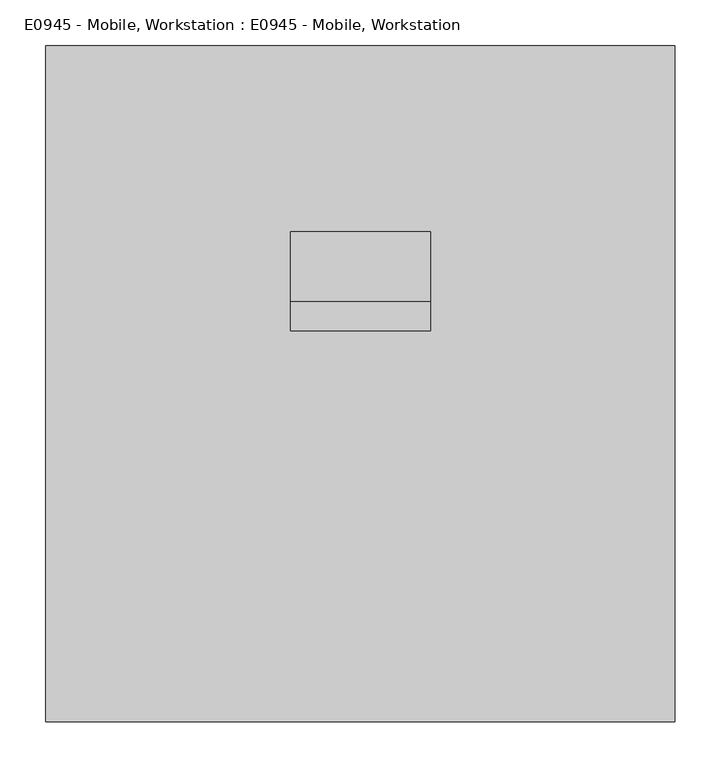
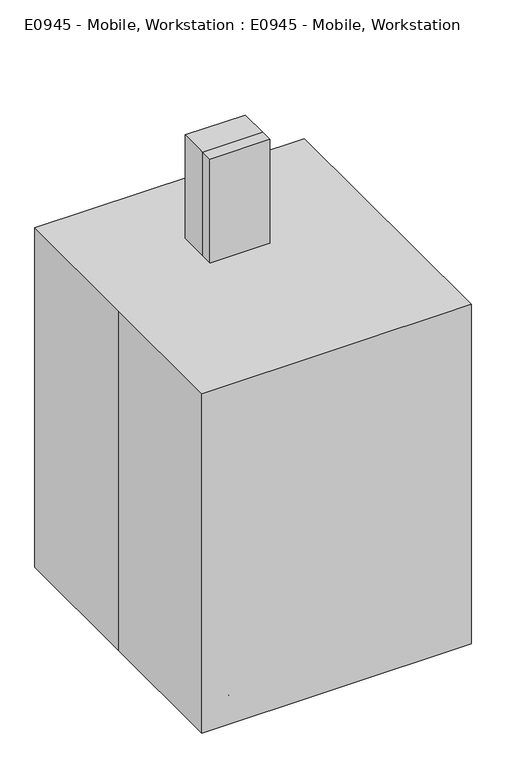
"""IFC4 building model written with IfcOpenShell, lengths in millimetres: proxy geometry, E0945 - Mobile, Workstation : E0945 - Mobile, Workstation."""

from ifc_helpers import new_model, si_unit, point, frame, frame_2d, origin, origin_with_axes, place, context, project, spatial, polyline, circle_curve, trimmed, segment, composite_curve, outline, extrude, faceted_brep, source, transform, mapped, element, save


def e0945_mobile_workstation_e0945_mobile_workstation_0c41a28f(model_context):
    return source(origin(), model_context, "Body", "SolidModel", [
        extrude(outline(polyline([(-196.85, 635.0), (58.0280886, 635.0), (58.0280886, 444.5), (-196.85, 609.6), (-196.85, 635.0)])), frame((57.15, 0.0, 0.0), z_axis=(1.0, 0.0, 0.0), x_axis=(0.0, 1.0, 0.0)), (0.0, 0.0, 1.0), 19.05),
        faceted_brep([(211.1375, -4.7625, 644.525), (211.1375, -4.7625, 639.7625), (211.1375, -255.5875, 639.7625), (211.1375, -255.5875, 644.525), (215.9, 0.0, 644.525), (215.9, -260.35, 644.525), (215.9, -260.35, 635.0), (215.9, 0.0, 635.0), (-211.1375, -255.5875, 639.7625), (-211.1375, -255.5875, 644.525), (-215.9, -260.35, 644.525), (-215.9, -260.35, 635.0), (-211.1375, -4.7625, 639.7625), (-211.1375, -4.7625, 644.525), (-215.9, 0.0, 644.525), (-215.9, 0.0, 635.0)], [[[0, 1, 2, 3]], [[4, 5, 6, 7]], [[3, 2, 8, 9]], [[6, 5, 10, 11]], [[9, 8, 12, 13]], [[11, 10, 14, 15]], [[1, 0, 13, 12]], [[5, 4, 14, 10], [0, 3, 9, 13]], [[4, 7, 15, 14]], [[7, 6, 11, 15]], [[2, 1, 12, 8]]]),
        extrude(outline(polyline([(-196.85, 635.0), (58.0280886, 635.0), (58.0280886, 444.5), (-196.85, 609.6), (-196.85, 635.0)])), frame((-76.2, 0.0, 0.0), z_axis=(1.0, 0.0, 0.0), x_axis=(0.0, 1.0, 0.0)), (0.0, 0.0, 1.0), 19.05),
        extrude(outline(polyline([(76.2, 89.7780886), (76.2, 58.0280886), (-76.2, 58.0280886), (-76.2, 89.7780886), (76.2, 89.7780886)])), frame((0.0, 0.0, 444.5), z_axis=(0.0, 0.0, 1.0), x_axis=(1.0, 0.0, 0.0)), (0.0, 0.0, 1.0), 749.3),
        extrude(outline(composite_curve([segment(polyline([(165.9780886, 1193.8), (165.9780886, 139.7), (62.2305834, 139.7)]), True, "CONTINUOUS"), segment(trimmed(circle_curve(frame_2d((29.5735373, 190.9359281)), 60.7585631), [point((62.2305834, 139.7))], [point((89.7780886, 182.7496596))], True, "CARTESIAN"), True, "CONTINUOUS"), segment(polyline([(89.7780886, 182.7496596), (89.7780886, 1193.8), (165.9780886, 1193.8)]), True, "CONTINUOUS")], self_intersect=False)), frame((-76.2, 0.0, 0.0), z_axis=(1.0, 0.0, 0.0), x_axis=(0.0, 1.0, 0.0)), (0.0, 0.0, 1.0), 152.4),
        extrude(outline(composite_curve([segment(trimmed(circle_curve(frame_2d((-215.9, 257.2471418)), 9.525), [point((-206.375, 257.2471418))], [point((-225.425, 257.2471418))], False, "CARTESIAN"), True, "CONTINUOUS"), segment(trimmed(circle_curve(frame_2d((-215.9, 257.2471418)), 9.525), [point((-225.425, 257.2471418))], [point((-206.375, 257.2471418))], False, "CARTESIAN"), True, "CONTINUOUS")], self_intersect=False)), frame((0.0, 0.0, 38.9774203), z_axis=(0.0, 0.0, 1.0), x_axis=(1.0, 0.0, 0.0)), (0.0, 0.0, 1.0), 49.9225797),
        extrude(outline(composite_curve([segment(trimmed(circle_curve(frame_2d((260.2876401, 38.1)), 38.1), [point((298.3876401, 38.1))], [point((222.1876401, 38.1))], False, "CARTESIAN"), True, "CONTINUOUS"), segment(trimmed(circle_curve(frame_2d((260.2876401, 38.1)), 38.1), [point((222.1876401, 38.1))], [point((298.3876401, 38.1))], False, "CARTESIAN"), True, "CONTINUOUS")], self_intersect=False)), frame((-206.375, 0.0, 0.0), z_axis=(1.0, 0.0, 0.0), x_axis=(0.0, 1.0, 0.0)), (0.0, 0.0, 1.0), 9.525),
        extrude(outline(composite_curve([segment(trimmed(circle_curve(frame_2d((260.35, 38.1)), 19.05), [point((279.4, 38.1))], [point((241.3, 38.1))], False, "CARTESIAN"), True, "CONTINUOUS"), segment(trimmed(circle_curve(frame_2d((260.35, 38.1)), 19.05), [point((241.3, 38.1))], [point((279.4, 38.1))], False, "CARTESIAN"), True, "CONTINUOUS")], self_intersect=False)), frame((-225.425, 0.0, 0.0), z_axis=(1.0, 0.0, 0.0), x_axis=(0.0, 1.0, 0.0)), (0.0, 0.0, 1.0), 19.05),
        extrude(outline(composite_curve([segment(trimmed(circle_curve(frame_2d((260.2876401, 38.1)), 38.1), [point((298.3876401, 38.1))], [point((222.1876401, 38.1))], False, "CARTESIAN"), True, "CONTINUOUS"), segment(trimmed(circle_curve(frame_2d((260.2876401, 38.1)), 38.1), [point((222.1876401, 38.1))], [point((298.3876401, 38.1))], False, "CARTESIAN"), True, "CONTINUOUS")], self_intersect=False)), frame((-234.95, 0.0, 0.0), z_axis=(1.0, 0.0, 0.0), x_axis=(0.0, 1.0, 0.0)), (0.0, 0.0, 1.0), 9.525),
        extrude(outline(composite_curve([segment(trimmed(circle_curve(frame_2d((-215.9, -257.2471418)), 9.525), [point((-206.375, -257.2471418))], [point((-225.425, -257.2471418))], False, "CARTESIAN"), True, "CONTINUOUS"), segment(trimmed(circle_curve(frame_2d((-215.9, -257.2471418)), 9.525), [point((-225.425, -257.2471418))], [point((-206.375, -257.2471418))], False, "CARTESIAN"), True, "CONTINUOUS")], self_intersect=False)), frame((0.0, 0.0, 38.9774203), z_axis=(0.0, 0.0, 1.0), x_axis=(1.0, 0.0, 0.0)), (0.0, 0.0, 1.0), 49.9225797),
        extrude(outline(composite_curve([segment(trimmed(circle_curve(frame_2d((-260.2876401, 38.1)), 38.1), [point((-298.3876401, 38.1))], [point((-222.1876401, 38.1))], False, "CARTESIAN"), True, "CONTINUOUS"), segment(trimmed(circle_curve(frame_2d((-260.2876401, 38.1)), 38.1), [point((-222.1876401, 38.1))], [point((-298.3876401, 38.1))], False, "CARTESIAN"), True, "CONTINUOUS")], self_intersect=False)), frame((-206.375, 0.0, 0.0), z_axis=(1.0, 0.0, 0.0), x_axis=(0.0, 1.0, 0.0)), (0.0, 0.0, 1.0), 9.525),
        extrude(outline(composite_curve([segment(trimmed(circle_curve(frame_2d((-260.35, 38.1)), 19.05), [point((-279.4, 38.1))], [point((-241.3, 38.1))], False, "CARTESIAN"), True, "CONTINUOUS"), segment(trimmed(circle_curve(frame_2d((-260.35, 38.1)), 19.05), [point((-241.3, 38.1))], [point((-279.4, 38.1))], False, "CARTESIAN"), True, "CONTINUOUS")], self_intersect=False)), frame((-225.425, 0.0, 0.0), z_axis=(1.0, 0.0, 0.0), x_axis=(0.0, 1.0, 0.0)), (0.0, 0.0, 1.0), 19.05),
        extrude(outline(composite_curve([segment(trimmed(circle_curve(frame_2d((-260.2876401, 38.1)), 38.1), [point((-298.3876401, 38.1))], [point((-222.1876401, 38.1))], False, "CARTESIAN"), True, "CONTINUOUS"), segment(trimmed(circle_curve(frame_2d((-260.2876401, 38.1)), 38.1), [point((-222.1876401, 38.1))], [point((-298.3876401, 38.1))], False, "CARTESIAN"), True, "CONTINUOUS")], self_intersect=False)), frame((-234.95, 0.0, 0.0), z_axis=(1.0, 0.0, 0.0), x_axis=(0.0, 1.0, 0.0)), (0.0, 0.0, 1.0), 9.525),
        extrude(outline(composite_curve([segment(trimmed(circle_curve(frame_2d((215.9, 257.2471418)), 9.525), [point((206.375, 257.2471418))], [point((225.425, 257.2471418))], False, "CARTESIAN"), True, "CONTINUOUS"), segment(trimmed(circle_curve(frame_2d((215.9, 257.2471418)), 9.525), [point((225.425, 257.2471418))], [point((206.375, 257.2471418))], False, "CARTESIAN"), True, "CONTINUOUS")], self_intersect=False)), frame((0.0, 0.0, 38.9774203), z_axis=(0.0, 0.0, 1.0), x_axis=(1.0, 0.0, 0.0)), (0.0, 0.0, 1.0), 49.9225797),
        extrude(outline(composite_curve([segment(trimmed(circle_curve(frame_2d((260.2876401, 38.1)), 38.1), [point((298.3876401, 38.1))], [point((222.1876401, 38.1))], False, "CARTESIAN"), True, "CONTINUOUS"), segment(trimmed(circle_curve(frame_2d((260.2876401, 38.1)), 38.1), [point((222.1876401, 38.1))], [point((298.3876401, 38.1))], False, "CARTESIAN"), True, "CONTINUOUS")], self_intersect=False)), frame((196.85, 0.0, 0.0), z_axis=(1.0, 0.0, 0.0), x_axis=(0.0, 1.0, 0.0)), (0.0, 0.0, 1.0), 9.525),
        extrude(outline(composite_curve([segment(trimmed(circle_curve(frame_2d((260.35, 38.1)), 19.05), [point((279.4, 38.1))], [point((241.3, 38.1))], False, "CARTESIAN"), True, "CONTINUOUS"), segment(trimmed(circle_curve(frame_2d((260.35, 38.1)), 19.05), [point((241.3, 38.1))], [point((279.4, 38.1))], False, "CARTESIAN"), True, "CONTINUOUS")], self_intersect=False)), frame((206.375, 0.0, 0.0), z_axis=(1.0, 0.0, 0.0), x_axis=(0.0, 1.0, 0.0)), (0.0, 0.0, 1.0), 19.05),
        extrude(outline(composite_curve([segment(trimmed(circle_curve(frame_2d((260.2876401, 38.1)), 38.1), [point((298.3876401, 38.1))], [point((222.1876401, 38.1))], False, "CARTESIAN"), True, "CONTINUOUS"), segment(trimmed(circle_curve(frame_2d((260.2876401, 38.1)), 38.1), [point((222.1876401, 38.1))], [point((298.3876401, 38.1))], False, "CARTESIAN"), True, "CONTINUOUS")], self_intersect=False)), frame((225.425, 0.0, 0.0), z_axis=(1.0, 0.0, 0.0), x_axis=(0.0, 1.0, 0.0)), (0.0, 0.0, 1.0), 9.525),
        extrude(outline(composite_curve([segment(trimmed(circle_curve(frame_2d((215.9, -257.2471418)), 9.525), [point((206.375, -257.2471418))], [point((225.425, -257.2471418))], False, "CARTESIAN"), True, "CONTINUOUS"), segment(trimmed(circle_curve(frame_2d((215.9, -257.2471418)), 9.525), [point((225.425, -257.2471418))], [point((206.375, -257.2471418))], False, "CARTESIAN"), True, "CONTINUOUS")], self_intersect=False)), frame((0.0, 0.0, 38.9774203), z_axis=(0.0, 0.0, 1.0), x_axis=(1.0, 0.0, 0.0)), (0.0, 0.0, 1.0), 49.9225797),
        extrude(outline(composite_curve([segment(trimmed(circle_curve(frame_2d((-260.2876401, 38.1)), 38.1), [point((-298.3876401, 38.1))], [point((-222.1876401, 38.1))], False, "CARTESIAN"), True, "CONTINUOUS"), segment(trimmed(circle_curve(frame_2d((-260.2876401, 38.1)), 38.1), [point((-222.1876401, 38.1))], [point((-298.3876401, 38.1))], False, "CARTESIAN"), True, "CONTINUOUS")], self_intersect=False)), frame((196.85, 0.0, 0.0), z_axis=(1.0, 0.0, 0.0), x_axis=(0.0, 1.0, 0.0)), (0.0, 0.0, 1.0), 9.525),
        extrude(outline(composite_curve([segment(trimmed(circle_curve(frame_2d((-260.35, 38.1)), 19.05), [point((-279.4, 38.1))], [point((-241.3, 38.1))], False, "CARTESIAN"), True, "CONTINUOUS"), segment(trimmed(circle_curve(frame_2d((-260.35, 38.1)), 19.05), [point((-241.3, 38.1))], [point((-279.4, 38.1))], False, "CARTESIAN"), True, "CONTINUOUS")], self_intersect=False)), frame((206.375, 0.0, 0.0), z_axis=(1.0, 0.0, 0.0), x_axis=(0.0, 1.0, 0.0)), (0.0, 0.0, 1.0), 19.05),
        extrude(outline(composite_curve([segment(trimmed(circle_curve(frame_2d((-260.2876401, 38.1)), 38.1), [point((-298.3876401, 38.1))], [point((-222.1876401, 38.1))], False, "CARTESIAN"), True, "CONTINUOUS"), segment(trimmed(circle_curve(frame_2d((-260.2876401, 38.1)), 38.1), [point((-222.1876401, 38.1))], [point((-298.3876401, 38.1))], False, "CARTESIAN"), True, "CONTINUOUS")], self_intersect=False)), frame((225.425, 0.0, 0.0), z_axis=(1.0, 0.0, 0.0), x_axis=(0.0, 1.0, 0.0)), (0.0, 0.0, 1.0), 9.525),
        extrude(outline(composite_curve([segment(polyline([(93.9865963, 192.9187071), (176.6628647, 292.6165602)]), True, "CONTINUOUS"), segment(trimmed(circle_curve(frame_2d((215.7665691, 260.189098)), 50.8), [point((176.6628647, 292.6165602))], [point((254.8702735, 227.7616359))], False, "CARTESIAN"), True, "CONTINUOUS"), segment(polyline([(254.8702735, 227.7616359), (152.4, 104.1945414), (152.4, -104.1945414), (254.8702735, -227.7616359)]), True, "CONTINUOUS"), segment(trimmed(circle_curve(frame_2d((215.7665691, -260.189098)), 50.8), [point((254.8702735, -227.7616359))], [point((176.6628647, -292.6165602))], False, "CARTESIAN"), True, "CONTINUOUS"), segment(polyline([(176.6628647, -292.6165602), (53.1141065, -143.6312929), (-53.1141065, -143.6312929), (-176.6628647, -292.6165602)]), True, "CONTINUOUS"), segment(trimmed(circle_curve(frame_2d((-215.7665691, -260.189098)), 50.8), [point((-176.6628647, -292.6165602))], [point((-254.8702735, -227.7616359))], False, "CARTESIAN"), True, "CONTINUOUS"), segment(polyline([(-254.8702735, -227.7616359), (-152.4, -104.1945414), (-152.4, 104.1945414), (-254.8702735, 227.7616359)]), True, "CONTINUOUS"), segment(trimmed(circle_curve(frame_2d((-215.7665691, 260.189098)), 50.8), [point((-254.8702735, 227.7616359))], [point((-176.6628647, 292.6165602))], False, "CARTESIAN"), True, "CONTINUOUS"), segment(polyline([(-176.6628647, 292.6165602), (-93.9865963, 192.9187071), (93.9865963, 192.9187071)]), True, "CONTINUOUS")], self_intersect=False)), frame((0.0, 0.0, 88.9), z_axis=(0.0, 0.0, 1.0), x_axis=(1.0, 0.0, 0.0)), (0.0, 0.0, 1.0), 50.8),
        extrude(outline(polyline([(-342.9, 368.3), (342.9, 368.3), (342.9, -368.3), (-342.9, -368.3), (-342.9, 0.0), (-342.9, 368.3)])), origin_with_axes(), (0.0, 0.0, 1.0), 914.4),
    ])


if __name__ == "__main__":
    model = new_model("IFC4")
    model_context = context("Model", 3, world=origin())
    ifc_project = project(units=[si_unit("LENGTHUNIT", "METRE", prefix="MILLI")], contexts=[model_context])
    site = spatial("IfcSite", under=ifc_project)
    building = spatial("IfcBuilding", under=site)
    placement = place(None, origin())
    e0945_mobile_workstation_e0945_mobile_workstation_shape = e0945_mobile_workstation_e0945_mobile_workstation_0c41a28f(model_context)
    element("IfcBuildingElementProxy", 1, Name="E0945 - Mobile, Workstation : E0945 - Mobile, Workstation", ObjectType="E0945 - Mobile, Workstation : E0945 - Mobile, Workstation", at=placement, inside=building, context=model_context, shape_type="MappedRepresentation", body=[
        mapped(e0945_mobile_workstation_e0945_mobile_workstation_shape, transform((0.0, 0.0, 0.0), x_axis=(1.0, 0.0, 0.0), y_axis=(0.0, 1.0, 0.0), z_axis=(0.0, 0.0, 1.0))),
    ])
    save(model, "model.ifc")

# Revit data of these elements
# Project information
#   Room Abbreviation = "TRET3"
#   Room Description = "Trauma/Resuscitation, Level I/II (TRET3)"
#   Sheets - Total = "6"
#   Project Issue Date = "Issue Date"
#   Project Status = "Project Status"
#   Client Name = "Owner"
#   Project Address = "Enter address here"
#   Project Name = "Project Name"
#   Project Number = "Project Number"
#   Publication Date = "30-Jan-15"
# Type "E0945 - Mobile, Workstation : E0945 - Mobile, Workstation"
#   Watts2 = "0"
#   Watts1 = "0"
#   Unit_Issue = "EA"
#   UTIL_6_Misc = "-"
#   UTIL_5_NonMedGas = "-"
#   UTIL_4_MiscGas = "-"
#   UTIL_3_MedGas = "-"
#   UTIL_2_Elec = "-"
#   UTIL_1_WaterDrain = "-"
#   Nomenclature = "Mobile, Workstation"
#   NSN = ""
#   Location [instance default] = ""
#   JSN = "E0945"
#   Fund_Source_VA = "-"
#   Fund_Source_Navy = "-"
#   Fund_Source_Army = "-"
#   Fund_Source_AF = "-"
#   ELEC_Volts2 = "0"
#   ELEC_Volts1 = "0"
#   ELEC_Phase2 = "0"
#   ELEC_Phase1 = "0"
#   ELEC_HertzSwitch = "0"
#   ELEC_HertzDependent = "0"
#   ELEC_Hertz = "0"
#   ELEC_Amps2 = "0"
#   ELEC_Amps1 = "0"
#   DetailDescription = ""
#   CAT_VA = "C"
#   CAT_Navy = "C"
#   CAT_IHS = "-"
#   CAT_Army = "C"
#   CAT_AF = "C"
#   BTUperhour = "0"
#   Weight_IP = 0
#   DIM_Width_IP = 2' - 3"
#   DIM_Height_IP = 3' - 0"
#   DIM_Depth_IP = 2' - 5"
# Element 1 (IfcBuildingElementProxy, "E0945 - Mobile, Workstation : E0945 - Mobile, Workstation")
#   Materials on its faces: "EquipSpace"
# Materials
#   "EquipSpace": class "Unassigned", colour RGB 221 217 195, transparency 0.5
